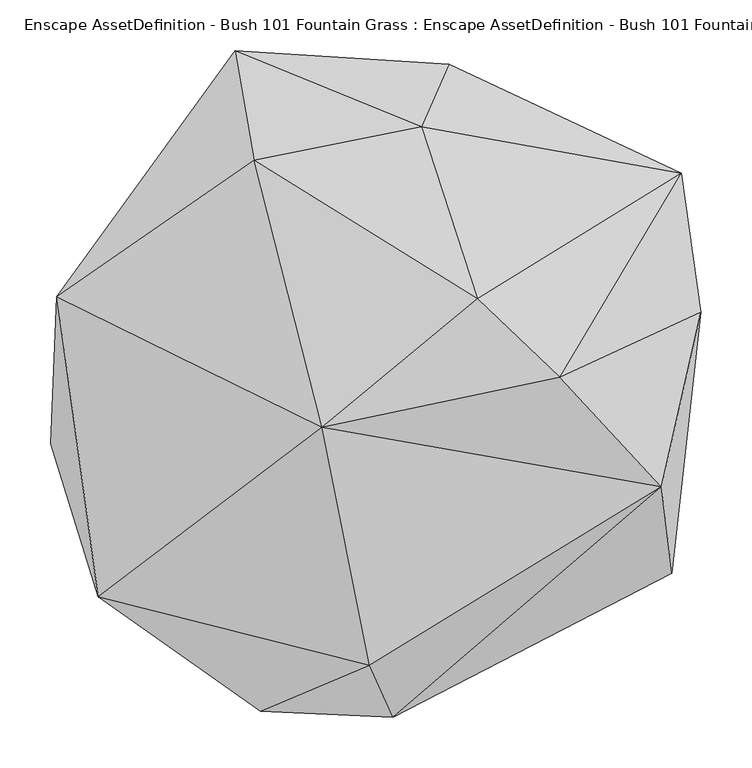
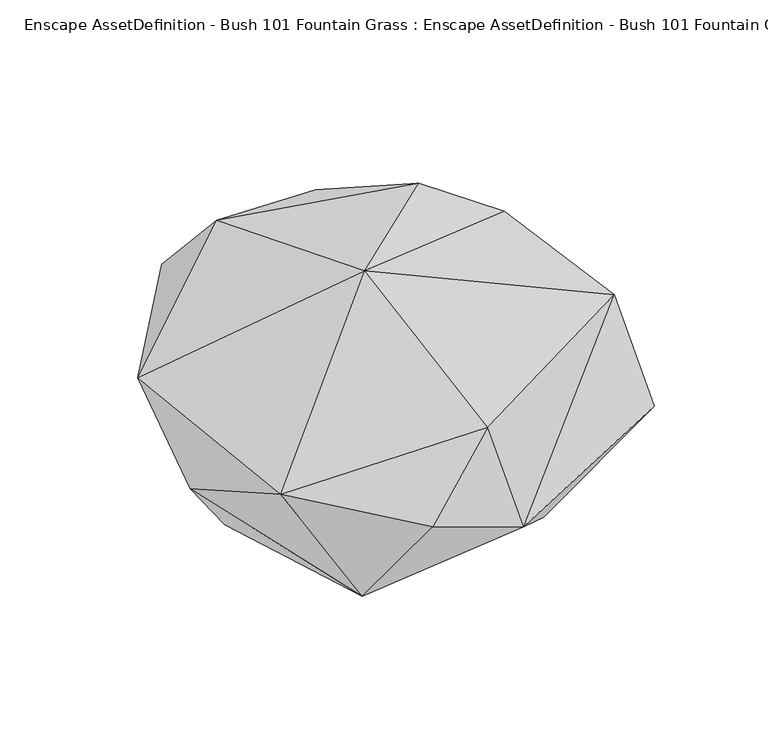
"""IFC4 building model written with IfcOpenShell, lengths in millimetres: geographic element geometry, Enscape AssetDefinition - Bush 101 Fountain Grass : Enscape AssetDefinition - Bush 101 Fountain Grass."""

from ifc_helpers import new_model, si_unit, origin, place, context, project, spatial, faceted_brep, source, transform, mapped, element, save


def enscape_assetdefinition_bush_101_fountain_grass_enscape_6dd3cd17(model_context):
    return source(origin(), model_context, "Body", "Brep", [
        faceted_brep([(290.726006, 204.2140067, 169.2969948), (310.0189865, 67.261003, 200.9090036), (285.8250141, -2.749, 94.4280028), (281.7150056, -188.9420003, 167.6100045), (271.3629901, -104.0429994, 293.4899926), (171.4809984, 3.548, 392.8869963), (155.6150019, -125.0769943, 0.0), (116.3929999, 116.6459993, 0.0), (7.5070001, -330.3700089, 161.4120007), (-15.9019995, -279.6109915, 293.5720086), (-62.4690019, -45.3479998, 411.6609991), (90.3849974, 80.6529969, 418.5400009), (-282.7430069, -211.9999975, 241.5329963), (-129.0519983, 216.7599946, 355.0690114), (-323.2310116, 82.4719965, 258.6530149), (-122.9199991, -324.5199919, 203.7439942), (-133.2180053, -162.0820016, 0.0), (-329.0739954, -61.5609996, 174.9459952), (-206.0199976, 63.9630035, 0.0), (-185.9450042, 241.3859963, 118.2629988), (-147.9399949, 324.2990077, 227.6110053), (35.6389992, 249.9070019, 324.76601), (31.4089991, 296.4580059, 111.9240001), (62.4630004, 311.1569881, 215.3590024), (-76.1179999, 157.0149958, 0.0)], [[[0, 1, 2]], [[1, 3, 2]], [[4, 3, 1]], [[4, 1, 5]], [[1, 0, 5]], [[2, 3, 6]], [[2, 6, 7]], [[2, 7, 0]], [[8, 3, 4]], [[3, 8, 6]], [[9, 8, 4]], [[10, 4, 5]], [[9, 4, 10]], [[10, 5, 11]], [[11, 5, 0]], [[12, 9, 10]], [[10, 11, 13]], [[10, 13, 14]], [[10, 14, 12]], [[12, 15, 9]], [[15, 8, 9]], [[8, 15, 16]], [[6, 8, 16]], [[15, 12, 16]], [[14, 17, 12]], [[17, 16, 12]], [[14, 18, 17]], [[19, 18, 14]], [[14, 13, 20]], [[20, 19, 14]], [[13, 11, 21]], [[21, 20, 13]], [[22, 19, 20]], [[21, 23, 20]], [[22, 20, 23]], [[19, 24, 18]], [[19, 22, 24]], [[22, 0, 7]], [[23, 0, 22]], [[24, 22, 7]], [[21, 0, 23]], [[11, 0, 21]], [[7, 6, 24]], [[18, 24, 6]], [[16, 18, 6]], [[17, 18, 16]]]),
    ])


if __name__ == "__main__":
    model = new_model("IFC4")
    model_context = context("Model", 3, world=origin())
    ifc_project = project(units=[si_unit("LENGTHUNIT", "METRE", prefix="MILLI")], contexts=[model_context])
    site = spatial("IfcSite", under=ifc_project)
    building = spatial("IfcBuilding", under=site)
    placement = place(None, origin())
    enscape_assetdefinition_bush_101_fountain_grass_enscape_shape = enscape_assetdefinition_bush_101_fountain_grass_enscape_6dd3cd17(model_context)
    element("IfcGeographicElement", 1, ObjectType="Enscape AssetDefinition - Bush 101 Fountain Grass : Enscape AssetDefinition - Bush 101 Fountain Grass", at=placement, inside=building, context=model_context, shape_type="MappedRepresentation", body=[
        mapped(enscape_assetdefinition_bush_101_fountain_grass_enscape_shape, transform((0.0, 0.0, 0.0), x_axis=(1.0, 0.0, 0.0), y_axis=(0.0, 1.0, 0.0), z_axis=(0.0, 0.0, 1.0))),
    ])
    save(model, "model.ifc")

# Revit data of these elements
# Type "Enscape AssetDefinition - Bush 101 Fountain Grass : Enscape AssetDefinition - Bush 101 Fountain Grass"
#   EnscapeAssetSource = "REMOTE"
#   EnscapeAssetId = "2a51c9c5-9004-4b2a-97bc-829b8068df40"
#   Height = 0.41854 m
#   EnscapeNativeAssetHeight = 0.41854 m
#   Default Elevation = 0
